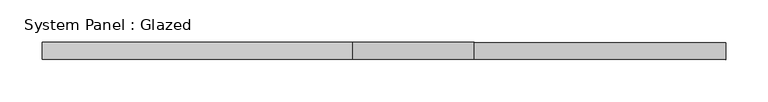
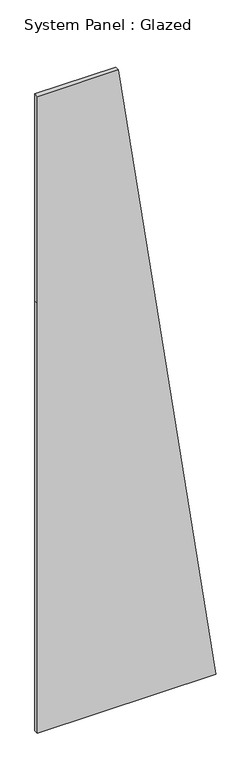
"""IFC4 building model written with IfcOpenShell, lengths in millimetres: plate geometry, System Panel : Glazed."""

from ifc_helpers import new_model, si_unit, frame, origin, place, context, project, spatial, polyline, outline, extrude, source, transform, mapped, element, save


def system_panel_glazed_cc08c4bb(model_context):
    return source(origin(), model_context, "Body", "SweptSolid", [
        extrude(outline(polyline([(0.0, -404.2975964), (0.0, 404.2975964), (2052.8288278, 106.7980927), (3050.0, -37.7136781), (3050.0, -404.2975964), (2060.0, -404.2975964), (0.0, -404.2975964)])), frame((0.0, 0.0, 0.0), z_axis=(0.0, 1.0, 0.0), x_axis=(0.0, 0.0, 1.0)), (0.0, 0.0, 1.0), 20.0),
    ])


if __name__ == "__main__":
    model = new_model("IFC4")
    model_context = context("Model", 3, world=origin())
    ifc_project = project(units=[si_unit("LENGTHUNIT", "METRE", prefix="MILLI")], contexts=[model_context])
    site = spatial("IfcSite", under=ifc_project)
    building = spatial("IfcBuilding", under=site)
    placement = place(None, origin())
    system_panel_glazed_shape = system_panel_glazed_cc08c4bb(model_context)
    element("IfcPlate", 1, ObjectType="System Panel : Glazed", at=placement, inside=building, context=model_context, shape_type="MappedRepresentation", body=[
        mapped(system_panel_glazed_shape, transform((0.0, 0.0, 0.0), x_axis=(1.0, 0.0, 0.0), y_axis=(0.0, 1.0, 0.0), z_axis=(0.0, 0.0, 1.0))),
    ])
    save(model, "model.ifc")

# Revit data of these elements
# Type "System Panel : Glazed"
#   COBie.Type = no
# Element 1 (IfcPlate, "System Panel : Glazed")
#   Materials on its faces: "Glass"
# Materials
#   "Glass": class "Glass", colour RGB 0 128 192, transparency 0.75, Description = "Soda Lime Glass", Cost = 0
